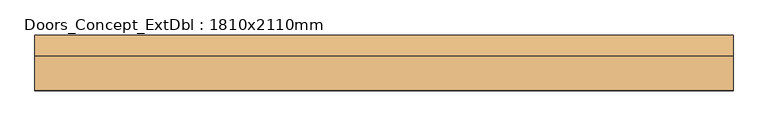
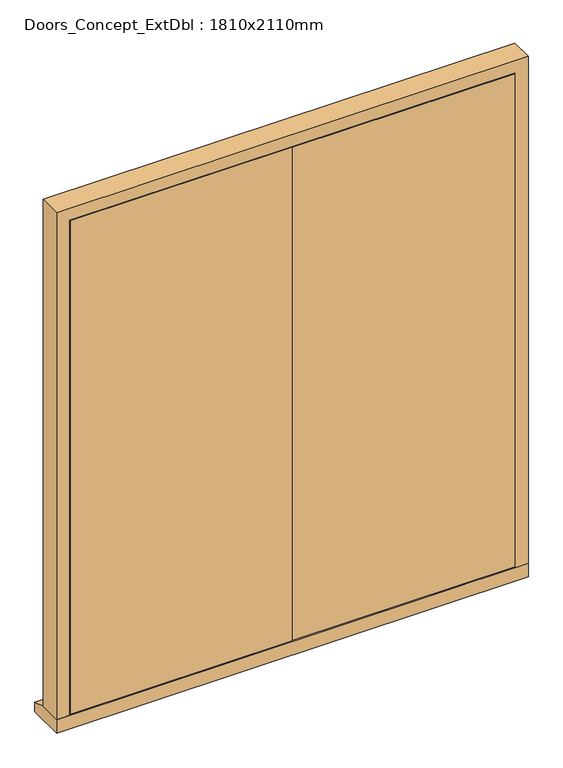
"""IFC4 building model written with IfcOpenShell, lengths in millimetres: door geometry, Doors_Concept_ExtDbl : 1810x2110mm."""

import ifcopenshell
import ifcopenshell.guid

model = None  # the IFC model being written
_history = None  # IfcOwnerHistory: only IFC2X3 demands one
_inside = {}  # id of a spatial element -> (the spatial element, [elements in it])
_under = {}  # id of a project, library or spatial element -> (it, [spatial elements below it])
_declared = {}  # id of a project -> (the project, [libraries it declares])
_typed = {}  # id of a type object -> (the type object, [elements of that type])
_made_of = {}  # id of a material, layer set ... -> (it, [elements and type objects made of it])


def new_model(schema):
    """Start an empty IFC model of exactly this schema.

    Asked for "IFC4X3", IfcOpenShell would pick the latest addendum, in which some entities
    have other attributes; the version numbers below select the first issue.
    IFC2X3 requires an IfcOwnerHistory on every rooted entity: one is made here for all.
    """
    global model, _history
    if schema == "IFC4X3":
        model = ifcopenshell.file(schema_version=(4, 3, 0, 0))
    else:
        model = ifcopenshell.file(schema=schema)
    _inside.clear()
    _under.clear()
    _declared.clear()
    _typed.clear()
    _made_of.clear()
    _history = None
    if model.schema == "IFC2X3":
        org = make("IfcOrganization", Name="unknown")
        user = make(
            "IfcPersonAndOrganization",
            ThePerson=make("IfcPerson", FamilyName="unknown"),
            TheOrganization=org,
        )
        app = make(
            "IfcApplication",
            ApplicationDeveloper=org,
            Version="unknown",
            ApplicationFullName="unknown",
            ApplicationIdentifier="unknown",
        )
        _history = make(
            "IfcOwnerHistory",
            OwningUser=user,
            OwningApplication=app,
            ChangeAction="ADDED",
            CreationDate=0,
        )
    return model


def make(cls, **values):
    """One entity of the class cls with the attributes given. An attribute that is None is left unset."""
    return model.create_entity(
        cls, **{name: value for name, value in values.items() if value is not None}
    )


def rooted(cls, **values):
    """An entity with a GlobalId (a new one), such as an element, a storey or a relation."""
    return make(cls, GlobalId=ifcopenshell.guid.new(), OwnerHistory=_history, **values)


def si_unit(unit_type, name, prefix=None):
    """IfcSIUnit, for example si_unit("LENGTHUNIT", "METRE", prefix="MILLI")."""
    return make("IfcSIUnit", UnitType=unit_type, Prefix=prefix, Name=name)


def assignment(units):
    """IfcUnitAssignment: the units of a project."""
    return None if units is None else make("IfcUnitAssignment", Units=units)


def point(xyz):
    """IfcCartesianPoint."""
    return None if xyz is None else make("IfcCartesianPoint", Coordinates=xyz)


def direction(xyz):
    """IfcDirection."""
    return None if xyz is None else make("IfcDirection", DirectionRatios=xyz)


def frame(location, z_axis=None, x_axis=None):
    """IfcAxis2Placement3D, a coordinate frame: its origin and axes. An axis left out is left unset."""
    return make(
        "IfcAxis2Placement3D",
        Location=point(location),
        Axis=direction(z_axis),
        RefDirection=direction(x_axis),
    )


def origin():
    """The frame at (0, 0, 0) with its axes left unset."""
    return frame((0.0, 0.0, 0.0))


def place(relative_to, where):
    """IfcLocalPlacement: puts the frame where relative to a parent placement (None: the world)."""
    return make(
        "IfcLocalPlacement", PlacementRelTo=relative_to, RelativePlacement=where
    )


def context(
    kind, dimensions, precision=None, world=None, true_north=None, identifier=None
):
    """IfcGeometricRepresentationContext, for example the 3D "Model" context."""
    return make(
        "IfcGeometricRepresentationContext",
        ContextIdentifier=identifier,
        ContextType=kind,
        CoordinateSpaceDimension=dimensions,
        Precision=precision,
        WorldCoordinateSystem=world,
        TrueNorth=true_north,
    )


def project(units=None, contexts=None):
    """IfcProject with its units and contexts."""
    return rooted(
        "IfcProject",
        Name="project",
        RepresentationContexts=contexts,
        UnitsInContext=assignment(units),
    )


def spatial(cls, under=None, at=None, **own):
    """A site, building, storey or space (cls), placed at a placement, below another one or the project."""
    s = rooted(cls, ObjectPlacement=at, **own)
    if under is not None:
        _under.setdefault(under.id(), (under, []))[1].append(s)
    return s


def polyline(points):
    """IfcPolyline through the points."""
    return make("IfcPolyline", Points=[point(p) for p in points])


def outline(outer, holes=None, kind="AREA"):
    """IfcArbitraryClosedProfileDef: a profile drawn as a closed curve; with holes, ...WithVoids."""
    if holes is None:
        return make("IfcArbitraryClosedProfileDef", ProfileType=kind, OuterCurve=outer)
    return make(
        "IfcArbitraryProfileDefWithVoids",
        ProfileType=kind,
        OuterCurve=outer,
        InnerCurves=holes,
    )


def extrude(swept, where, along, depth):
    """IfcExtrudedAreaSolid: the profile swept, set in the frame where, extruded along a direction by depth."""
    return make(
        "IfcExtrudedAreaSolid",
        SweptArea=swept,
        Position=where,
        ExtrudedDirection=direction(along),
        Depth=depth,
    )


def faces_of(points, faces, orient=None, outer=None):
    """IfcFace entities. A face is a list of loops; a loop is a list of indices into points, from 0.

    orient and outer hold one flag for each loop. By default every Orientation is true, the
    first loop of a face is its IfcFaceOuterBound and the others are IfcFaceBound.
    """
    made = []
    for i, loops in enumerate(faces):
        bounds = []
        for j, loop in enumerate(loops):
            is_outer = j == 0 if outer is None else outer[i][j]
            bounds.append(
                make(
                    "IfcFaceOuterBound" if is_outer else "IfcFaceBound",
                    Bound=make("IfcPolyLoop", Polygon=[points[k] for k in loop]),
                    Orientation=True if orient is None else orient[i][j],
                )
            )
        made.append(make("IfcFace", Bounds=bounds))
    return made


def faceted_brep(points, faces, orient=None, outer=None, voids=None):
    """IfcFacetedBrep: a solid bounded by flat faces; with voids (closed shells), ...WithVoids."""
    shared = [point(p) for p in points]
    hull = make("IfcClosedShell", CfsFaces=faces_of(shared, faces, orient, outer))
    if voids is None:
        return make("IfcFacetedBrep", Outer=hull)
    return make(
        "IfcFacetedBrepWithVoids",
        Outer=hull,
        Voids=[
            make(cls, CfsFaces=faces_of(shared, fs, o, b)) for cls, fs, o, b in voids
        ],
    )


def shape(context_of_items, identifier, shape_type, items):
    """IfcShapeRepresentation: the items that make up one representation, for example the "Body"."""
    return make(
        "IfcShapeRepresentation",
        ContextOfItems=context_of_items,
        RepresentationIdentifier=identifier,
        RepresentationType=shape_type,
        Items=items,
    )


def source(mapping_origin, context_of_items, identifier, shape_type, items):
    """IfcRepresentationMap: a shape defined once, which mapped items show again and again."""
    return make(
        "IfcRepresentationMap",
        MappingOrigin=mapping_origin,
        MappedRepresentation=shape(context_of_items, identifier, shape_type, items),
    )


def transform(
    local_origin,
    x_axis=None,
    y_axis=None,
    z_axis=None,
    scale=None,
    scale2=None,
    scale3=None,
    uniform=True,
):
    """IfcCartesianTransformationOperator3D, or its non-uniform kind. x_axis, y_axis, z_axis: its Axis1, 2, 3."""
    if uniform:
        return make(
            "IfcCartesianTransformationOperator3D",
            Axis1=direction(x_axis),
            Axis2=direction(y_axis),
            LocalOrigin=point(local_origin),
            Scale=scale,
            Axis3=direction(z_axis),
        )
    return make(
        "IfcCartesianTransformationOperator3DnonUniform",
        Axis1=direction(x_axis),
        Axis2=direction(y_axis),
        LocalOrigin=point(local_origin),
        Scale=scale,
        Axis3=direction(z_axis),
        Scale2=scale2,
        Scale3=scale3,
    )


def mapped(mapping_source, mapping_target):
    """IfcMappedItem: shows the shape of a source again, moved by a transform."""
    return make(
        "IfcMappedItem", MappingSource=mapping_source, MappingTarget=mapping_target
    )


def made_of(thing, what):
    """Note that an element or type object is made of a material, layer set ...; save() writes the relation."""
    if what is not None:
        _made_of.setdefault(what.id(), (what, []))[1].append(thing)
    return thing


def element(
    cls,
    number,
    at=None,
    inside=None,
    cuts=None,
    type_object=None,
    material=None,
    context=None,
    identifier="Body",
    shape_type=None,
    held_by="IfcProductDefinitionShape",
    body=None,
    shapes=None,
    **own,
):
    """One element of the class cls, such as IfcWall. Its Tag is "e" and its number.

    at: its placement. inside: the storey or other place that contains it. cuts: it is an
    opening in that element (IfcRelVoidsElement). A single representation is given by context,
    identifier, shape_type and body (its items); several are given by shapes. held_by: the class
    of the entity that holds the representations. save() writes the other relations.
    """
    e = rooted(cls, Tag="e%d" % number, ObjectPlacement=at, **own)
    if body is not None:
        shapes = [shape(context, identifier, shape_type, body)]
    if shapes is not None:
        e.Representation = make(held_by, Representations=shapes)
    if inside is not None:
        _inside.setdefault(inside.id(), (inside, []))[1].append(e)
    if cuts is not None:
        rooted(
            "IfcRelVoidsElement", RelatingBuildingElement=cuts, RelatedOpeningElement=e
        )
    if type_object is not None:
        _typed.setdefault(type_object.id(), (type_object, []))[1].append(e)
    return made_of(e, material)


def aggregate(whole, parts):
    """IfcRelAggregates: a whole, such as a stair, and the parts it consists of."""
    return rooted("IfcRelAggregates", RelatingObject=whole, RelatedObjects=parts)


def save(model, path):
    """Write the relations noted so far, then the file.

    IfcRelAggregates (storeys below a building ...), IfcRelContainedInSpatialStructure (elements
    in a storey), IfcRelDefinesByType, IfcRelAssociatesMaterial and IfcRelDeclares: one each for
    every whole, place, type object, material and project.
    """
    for whole, parts in _under.values():
        aggregate(whole, parts)
    for where, things in _inside.values():
        rooted(
            "IfcRelContainedInSpatialStructure",
            RelatedElements=things,
            RelatingStructure=where,
        )
    for kind, things in _typed.values():
        rooted("IfcRelDefinesByType", RelatedObjects=things, RelatingType=kind)
    for what, things in _made_of.values():
        rooted("IfcRelAssociatesMaterial", RelatedObjects=things, RelatingMaterial=what)
    for by, libraries in _declared.values():
        rooted("IfcRelDeclares", RelatingContext=by, RelatedDefinitions=libraries)
    model.write(path)


def doors_concept_extdbl_1810x2110mm_b9f5cbc2(model_context):
    return source(origin(), model_context, "Body", "SolidModel", [
        faceted_brep([(834.5, 137.25, 54.5), (905.0, 137.25, 54.5), (905.0, 48.25, 54.5), (856.5, 48.25, 54.5), (856.5, 95.25, 54.5), (834.5, 95.25, 54.5), (834.5, 137.25, 2039.5), (-834.5, 137.25, 2039.5), (-834.5, 137.25, 54.5), (-905.0, 137.25, 54.5), (-905.0, 137.25, 2110.0), (905.0, 137.25, 2110.0), (905.0, 48.25, 2110.0), (-905.0, 48.25, 2110.0), (-905.0, 48.25, 54.5), (-856.5, 48.25, 54.5), (-856.5, 48.25, 2061.5), (856.5, 48.25, 2061.5), (856.5, 95.25, 2061.5), (-856.5, 95.25, 2061.5), (-856.5, 95.25, 54.5), (-834.5, 95.25, 54.5), (-834.5, 95.25, 2039.5), (834.5, 95.25, 2039.5)], [[[0, 1, 2, 3, 4, 5]], [[1, 0, 6, 7, 8, 9, 10, 11]], [[2, 1, 11, 12]], [[3, 2, 12, 13, 14, 15, 16, 17]], [[4, 3, 17, 18]], [[5, 4, 18, 19, 20, 21, 22, 23]], [[0, 5, 23, 6]], [[7, 22, 21, 8]], [[8, 21, 20, 15, 14, 9]], [[13, 10, 9, 14]], [[19, 16, 15, 20]], [[12, 11, 10, 13]], [[18, 17, 16, 19]], [[6, 23, 22, 7]]]),
        extrude(outline(polyline([(48.25, 0.0), (48.25, 54.5), (137.25, 54.5), (192.25, 38.5947221), (192.25, 0.0), (48.25, 0.0)])), frame((-905.0, 0.0, 0.0), z_axis=(1.0, 0.0, 0.0), x_axis=(0.0, 1.0, 0.0)), (0.0, 0.0, 1.0), 1810.0),
        extrude(outline(polyline([(853.5, 48.25), (1.5, 48.25), (1.5, 92.25), (853.5, 92.25), (853.5, 48.25)])), frame((0.0, 0.0, 58.5), z_axis=(0.0, 0.0, 1.0), x_axis=(1.0, 0.0, 0.0)), (0.0, 0.0, 1.0), 2000.0),
        extrude(outline(polyline([(-1.5, 48.25), (-853.5, 48.25), (-853.5, 92.25), (-1.5, 92.25), (-1.5, 48.25)])), frame((0.0, 0.0, 58.5), z_axis=(0.0, 0.0, 1.0), x_axis=(1.0, 0.0, 0.0)), (0.0, 0.0, 1.0), 2000.0),
    ])


if __name__ == "__main__":
    model = new_model("IFC4")
    model_context = context("Model", 3, world=origin())
    ifc_project = project(units=[si_unit("LENGTHUNIT", "METRE", prefix="MILLI")], contexts=[model_context])
    site = spatial("IfcSite", under=ifc_project)
    building = spatial("IfcBuilding", under=site)
    placement = place(None, origin())
    doors_concept_extdbl_1810x2110mm_shape = doors_concept_extdbl_1810x2110mm_b9f5cbc2(model_context)
    element("IfcDoor", 1, ObjectType="Doors_Concept_ExtDbl : 1810x2110mm", at=placement, inside=building, context=model_context, shape_type="MappedRepresentation", body=[
        mapped(doors_concept_extdbl_1810x2110mm_shape, transform((0.0, 0.0, 0.0), x_axis=(1.0, 0.0, 0.0), y_axis=(0.0, 1.0, 0.0), z_axis=(0.0, 0.0, 1.0))),
    ])
    save(model, "model.ifc")

# Revit data of these elements
# Type "Doors_Concept_ExtDbl : 1810x2110mm"
#   Type Mark = "47"
#   Type Comments = "External Double"
#   Operation = "DoubleDoorSingleSwing"
#   Construction Type Id = "GSP4R"
#   Keynote = "L10"
#   Analytic Construction = "1/8 in Pilkington single glazing"
#   Visual Light Transmittance = 0.9
#   Thickness = 44 mm
#   Solar Heat Gain Coefficient = 0.78
#   Rough Width = 1810 mm
#   Rough Height = 2110 mm
#   Heat Transfer Coefficient (U) = 3.6886 W/(m²·K)
#   FrameWidth = 42 mm
#   FrameOffset - External = 25 mm
#   Height = 2110 mm
#   Width = 1810 mm
#   Function = 1
#   Material Door = Concept
#   Material Frame = Concept
#   Wall Closure = (empty or 0)
# Element 1 (IfcDoor, "Doors_Concept_ExtDbl : 1810x2110mm")
#   Materials on its faces: "Concept"
# Materials
#   "Concept": class "Miscellaneous", colour RGB 128 128 255, transparency 0.5
